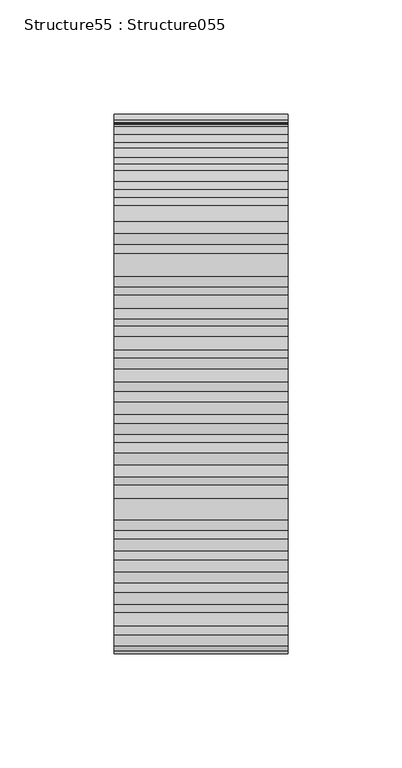
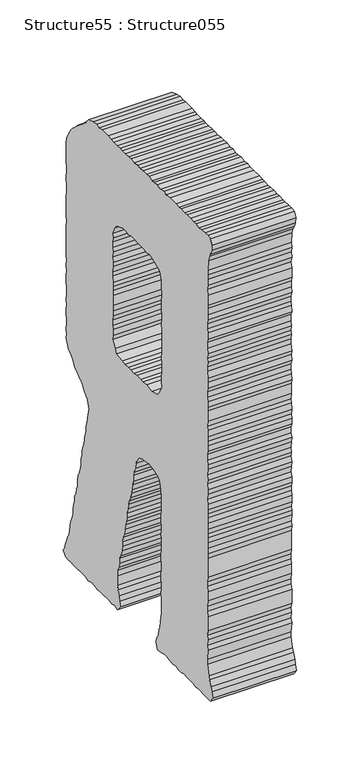
"""IFC4 building model written with IfcOpenShell, lengths in millimetres: proxy geometry, Structure55 : Structure055."""

from ifc_helpers import new_model, si_unit, frame, origin, place, context, project, spatial, polyline, outline, extrude, source, transform, mapped, element, save


def structure55_structure055_96c68484(model_context):
    return source(origin(), model_context, "Body", "SweptSolid", [
        extrude(outline(polyline([(253600.0102866, 3899.7046941), (253600.0102866, 3894.4030808), (253600.6007811, 3890.320967), (253600.0102866, 3884.4609514), (253600.0102866, 3880.3627915), (253599.4262106, 3876.263027), (253600.6007811, 3870.4030114), (253600.0102866, 3866.8776953), (253600.0102866, 3856.9179152), (253600.6007811, 3851.6612309), (253600.0102866, 3846.9757858), (253600.0102866, 3842.8583706), (253599.4262106, 3838.1761347), (253600.6007811, 3832.8921721), (253599.4262106, 3827.6162325), (253600.0102866, 3823.5341187), (253600.6007811, 3818.2309008), (253599.4262106, 3810.0474179), (253599.4262106, 3804.1890069), (253600.6007811, 3800.0876378), (253599.4262106, 3794.8309535), (253600.6007811, 3790.7039107), (253600.6007811, 3785.4456218), (253599.4262106, 3781.9299333), (253599.4262106, 3777.2444882), (253600.6007811, 3771.3860772), (253599.4262106, 3766.684586), (253600.6007811, 3762.5848215), (253596.5026212, 3753.8012165), (253592.3932291, 3751.4424479), (253589.4680351, 3747.9428055), (253586.5428411, 3743.2332913), (253582.4430766, 3739.7416719), (253579.5098596, 3737.9750024), (253575.4084905, 3734.47536), (253571.892802, 3729.7738688), (253568.9579804, 3726.2742264), (253566.0327864, 3723.9154578), (253563.6916685, 3716.2887726), (253566.0327864, 3706.9130685), (253567.1993339, 3701.0723082), (253568.367486, 3696.9709391), (253568.367486, 3691.6869765), (253570.1341555, 3687.587212), (253571.308726, 3683.4858429), (253571.892802, 3678.2018803), (253573.6514486, 3674.1277895), (253574.8163914, 3670.0007467), (253575.4084905, 3665.3265338), (253576.5750379, 3660.6250426), (253576.5750379, 3654.7842823), (253578.9257835, 3646.557475), (253581.2685061, 3641.8832621), (253582.4430766, 3636.6153456), (253581.8493729, 3631.3410106), (253583.601601, 3627.8397636), (253584.1920955, 3622.555801), (253586.5428411, 3619.0385079), (253587.1188941, 3613.772196), (253588.2934646, 3609.6547808), (253589.4680351, 3604.3964919), (253589.4680351, 3600.2967274), (253590.6442102, 3595.5872132), (253592.9837235, 3590.3289243), (253594.1615032, 3585.0706354), (253595.9105221, 3576.2693797), (253598.2532447, 3572.7440636), (253599.4262106, 3568.0682461), (253601.1848571, 3564.54293), (253602.3530092, 3559.2669905), (253604.7021502, 3556.3417965), (253601.1848571, 3551.6675836), (253596.5026212, 3551.0658569), (253592.9837235, 3551.6675836), (253588.2934646, 3551.0658569), (253583.0271526, 3551.0658569), (253578.3336845, 3551.6675836), (253569.5404518, 3551.6675836), (253565.4406874, 3550.4833855), (253559.5822763, 3551.6675836), (253556.0730063, 3551.6675836), (253551.3795382, 3550.4833855), (253545.5307548, 3551.0658569), (253532.0472632, 3551.0658569), (253527.9458941, 3550.4833855), (253523.836502, 3551.6675836), (253519.1606845, 3550.4833855), (253514.4704255, 3556.3417965), (253516.2194444, 3560.441561), (253516.8115435, 3565.1254015), (253517.986114, 3570.4109687), (253519.1606845, 3573.9266571), (253519.1606845, 3583.2863152), (253519.1606845, 3588.5702778), (253516.8115435, 3592.6700423), (253516.2194444, 3596.7698067), (253515.644996, 3602.0280957), (253513.2958551, 3606.1551384), (253512.1180754, 3611.4134274), (253511.5436269, 3616.0972679), (253510.9531325, 3620.7971545), (253510.3690565, 3625.472972), (253508.0263339, 3629.5984101), (253507.4454671, 3634.856699), (253506.8517634, 3639.5405396), (253505.0947215, 3644.2420307), (253503.928174, 3648.3161216), (253503.928174, 3652.4431643), (253502.7519989, 3657.7014533), (253501.5774284, 3662.3836892), (253499.8284095, 3667.0851803), (253498.6426068, 3670.5848228), (253496.8919833, 3675.8687854), (253496.3111165, 3679.9701544), (253495.1349414, 3685.2444894), (253493.9603709, 3689.3458585), (253493.9603709, 3695.2122926), (253492.7922188, 3698.711935), (253491.0255493, 3703.4134261), (253489.8509788, 3709.2718371), (253485.7496097, 3716.8985223), (253478.7246512, 3719.8140887), (253472.8662402, 3719.8140887), (253469.3585748, 3720.9726131), (253463.4905361, 3719.8140887), (253455.2894025, 3717.4729707), (253452.3561855, 3713.9556777), (253450.6071666, 3706.9130685), (253449.4293869, 3701.6547796), (253449.4293869, 3688.1873341), (253450.6071666, 3683.4858429), (253450.6071666, 3677.6274319), (253449.4293869, 3672.9435914), (253450.013463, 3668.2437048), (253450.6071666, 3664.7440624), (253450.013463, 3660.0682449), (253450.013463, 3654.1841602), (253449.4293869, 3650.1004418), (253450.6071666, 3644.8245022), (253450.6071666, 3640.114988), (253450.013463, 3636.6153456), (253449.4293869, 3631.915459), (253450.6071666, 3626.0554434), (253450.6071666, 3621.3732075), (253449.4293869, 3617.2718384), (253449.4293869, 3613.1720739), (253450.6071666, 3607.8961343), (253449.4293869, 3602.6298224), (253450.013463, 3597.9540049), (253450.013463, 3594.4286888), (253449.4293869, 3589.1527492), (253450.6071666, 3585.0706354), (253451.7817371, 3574.5107332), (253453.530756, 3570.9854171), (253454.7069311, 3565.1254015), (253457.0480491, 3561.6257591), (253458.2242242, 3556.3417965), (253455.8734786, 3550.4833855), (253450.013463, 3551.0658569), (253445.331227, 3552.242032), (253441.2218349, 3552.242032), (253437.1204658, 3551.6675836), (253431.8557585, 3551.0658569), (253427.1622903, 3551.6675836), (253423.0609212, 3551.0658569), (253418.3690577, 3551.0658569), (253414.2773162, 3552.242032), (253409.5838481, 3551.6675836), (253399.6272772, 3551.6675836), (253394.9418321, 3551.0658569), (253390.8420676, 3551.6675836), (253380.8758691, 3551.6675836), (253376.7841276, 3551.0658569), (253372.6827585, 3551.0658569), (253368.5733664, 3556.3417965), (253370.3223853, 3561.6257591), (253371.508188, 3565.7094775), (253373.8396783, 3570.9854171), (253375.0158534, 3574.5107332), (253377.358576, 3583.8864372), (253377.358576, 3588.5702778), (253376.1904239, 3597.9540049), (253377.358576, 3602.0280957), (253376.7841276, 3607.8961343), (253377.358576, 3612.0135494), (253376.1904239, 3616.69739), (253376.1904239, 3630.1824862), (253377.358576, 3634.856699), (253377.358576, 3639.5405396), (253376.7841276, 3645.4262289), (253376.7841276, 3654.1841602), (253377.358576, 3658.8840468), (253377.358576, 3663.5598643), (253376.7841276, 3668.2437048), (253376.7841276, 3686.4030139), (253376.1904239, 3691.0868544), (253376.7841276, 3695.786741), (253376.1904239, 3701.6547796), (253376.1904239, 3706.3289925), (253376.7841276, 3709.8559132), (253376.1904239, 3714.5301261), (253376.1904239, 3720.4158154), (253376.7841276, 3725.0996559), (253376.7841276, 3729.1737467), (253376.1904239, 3733.2991849), (253376.1904239, 3738.5574738), (253377.358576, 3742.6748889), (253376.7841276, 3747.9428055), (253376.1904239, 3752.6170184), (253377.358576, 3757.8753073), (253376.7841276, 3761.418274), (253377.358576, 3766.1021146), (253376.7841276, 3771.9605256), (253376.1904239, 3776.6427615), (253377.358576, 3780.1616592), (253377.358576, 3786.0280932), (253376.1904239, 3789.5293402), (253376.1904239, 3794.8309535), (253376.7841276, 3798.9050443), (253376.1904239, 3803.5872802), (253376.7841276, 3809.4729695), (253377.358576, 3812.9726119), (253376.7841276, 3818.2309008), (253376.7841276, 3828.2163546), (253376.1904239, 3831.732043), (253376.7841276, 3836.9919366), (253377.358576, 3841.0900965), (253377.358576, 3846.3772683), (253376.1904239, 3850.4754282), (253376.7841276, 3855.7353217), (253376.1904239, 3859.8591552), (253377.358576, 3865.7015202), (253377.358576, 3870.4030114), (253376.7841276, 3875.0772243), (253377.358576, 3878.5784713), (253376.7841276, 3883.2863809), (253377.358576, 3887.9621984), (253377.358576, 3893.822214), (253376.1904239, 3897.3475301), (253376.7841276, 3903.2059411), (253377.358576, 3906.7328618), (253377.358576, 3911.4054701), (253376.1904239, 3916.0909152), (253376.7841276, 3920.7908018), (253376.7841276, 3926.6492128), (253376.1904239, 3930.1745289), (253376.1904239, 3939.5325823), (253377.358576, 3944.8165449), (253376.1904239, 3949.4923624), (253376.7841276, 3954.7506513), (253376.1904239, 3959.4617701), (253376.7841276, 3963.5615346), (253375.6063479, 3973.5197101), (253374.4317774, 3978.2035506), (253372.0906594, 3981.7208437), (253370.3223853, 3986.4046842), (253369.7415185, 3991.6806238), (253372.0906594, 3996.390138), (253376.7841276, 3996.9645864), (253380.8758691, 3996.9645864), (253386.7406985, 3996.390138), (253390.2515731, 3996.390138), (253395.5355357, 3996.9645864), (253399.6272772, 3996.390138), (253404.3095131, 3996.9645864), (253409.5838481, 3996.9645864), (253413.6932402, 3996.390138), (253418.9627614, 3996.9645864), (253422.4784498, 3996.390138), (253427.1622903, 3996.9645864), (253436.5460174, 3996.9645864), (253442.3964054, 3996.390138), (253445.9136985, 3997.5486624), (253451.1880334, 3996.390138), (253456.45595, 3997.5486624), (253461.1478136, 3996.9645864), (253464.6651066, 3996.390138), (253469.3585748, 3997.5486624), (253473.4583392, 3996.9645864), (253478.7246512, 3997.5486624), (253483.4068871, 3996.9645864), (253487.5162792, 3997.5486624), (253493.3666672, 3996.390138), (253498.0601354, 3996.9645864), (253501.5774284, 3996.9645864), (253507.4454671, 3996.390138), (253512.1180754, 3996.390138), (253515.0625246, 3996.9645864), (253519.7367375, 3996.390138), (253525.6047761, 3996.390138), (253529.1124416, 3996.9645864), (253533.8059097, 3997.5486624), (253543.7656898, 3997.5486624), (253547.8638497, 3996.9645864), (253552.5573179, 3997.5486624), (253557.8236298, 3996.390138), (253564.8469837, 3994.0233463), (253568.367486, 3989.9460463), (253571.892802, 3987.0048063), (253575.4084905, 3982.8793681), (253580.0827034, 3979.9621971), (253583.0271526, 3977.6194746), (253585.950742, 3974.1214368), (253590.0601341, 3970.5768654), (253592.3932291, 3967.6789497), (253595.9105221, 3962.9774586), (253599.4262106, 3955.360401), (253600.0102866, 3951.2606365), (253600.0102866, 3941.8753048), (253600.6007811, 3936.0345445), (253600.6007811, 3932.4899731), (253599.4262106, 3927.8077372), (253599.4262106, 3923.1319197), (253600.6007811, 3918.4480792), (253599.4262106, 3907.888177), (253599.4262106, 3903.2059411), (253600.0102866, 3899.7046941)]), holes=[polyline([(253472.8662402, 3794.8309535), (253478.7246512, 3794.2292268), (253482.2323166, 3794.8309535), (253488.1003553, 3794.8309535), (253493.3666672, 3793.6451507), (253498.0601354, 3794.2292268), (253501.5774284, 3794.2292268), (253507.4454671, 3793.6451507), (253511.5436269, 3794.8309535), (253520.3288366, 3795.960595), (253522.0874831, 3800.0876378), (253526.1872476, 3806.5317294), (253525.6047761, 3810.6298893), (253525.6047761, 3816.4883003), (253526.1872476, 3820.015221), (253526.1872476, 3825.2911606), (253525.6047761, 3829.374879), (253525.6047761, 3834.0474873), (253525.0110725, 3839.9331766), (253525.0110725, 3849.3008577), (253525.6047761, 3854.0007442), (253525.0110725, 3858.1021133), (253525.0110725, 3862.2018778), (253526.1872476, 3867.4601667), (253526.1872476, 3871.5599312), (253525.6047761, 3876.8438938), (253525.6047761, 3880.9452629), (253526.1872476, 3885.6210804), (253525.6047761, 3890.905043), (253526.1872476, 3895.0048075), (253526.1872476, 3900.2887701), (253525.6047761, 3904.3901392), (253526.1872476, 3908.46423), (253523.252426, 3915.5068392), (253519.7367375, 3919.0321552), (253510.9531325, 3922.5494483), (253506.2596643, 3922.5494483), (253502.7519989, 3921.3748778), (253498.0601354, 3922.5494483), (253483.4068871, 3922.5494483), (253477.5564991, 3921.9733953), (253474.0408107, 3921.3748778), (253469.3585748, 3922.5494483), (253464.6651066, 3921.3748778), (253456.45595, 3918.4480792), (253452.9482846, 3916.0909152), (253450.6071666, 3909.0627475), (253450.6071666, 3904.9645876), (253449.4293869, 3894.4030808), (253450.6071666, 3890.320967), (253450.6071666, 3880.3627915), (253449.4293869, 3876.8438938), (253450.013463, 3871.5599312), (253450.6071666, 3867.4601667), (253449.4293869, 3861.6178018), (253450.013463, 3858.1021133), (253450.013463, 3839.9331766), (253450.6071666, 3834.6588416), (253449.4293869, 3830.5574726), (253449.4293869, 3825.849563), (253450.013463, 3820.5896694), (253450.6071666, 3816.4883003), (253450.6071666, 3811.7884138), (253450.013463, 3805.9476534), (253452.9482846, 3800.0876378), (253455.8734786, 3795.960595), (253464.6651066, 3793.6451507), (253472.8662402, 3794.8309535)])]), frame((-38594.2176606, 0.0, 0.0), z_axis=(1.0, 0.0, 0.0), x_axis=(0.0, 1.0, 0.0)), (0.0, 0.0, 1.0), 76.2),
    ])


if __name__ == "__main__":
    model = new_model("IFC4")
    model_context = context("Model", 3, world=origin())
    ifc_project = project(units=[si_unit("LENGTHUNIT", "METRE", prefix="MILLI")], contexts=[model_context])
    site = spatial("IfcSite", under=ifc_project)
    building = spatial("IfcBuilding", under=site)
    placement = place(None, origin())
    structure55_structure055_shape = structure55_structure055_96c68484(model_context)
    element("IfcBuildingElementProxy", 1, Name="Structure55 : Structure055", ObjectType="Structure55 : Structure055", at=placement, inside=building, context=model_context, shape_type="MappedRepresentation", body=[
        mapped(structure55_structure055_shape, transform((0.0, 0.0, 0.0), x_axis=(1.0, 0.0, 0.0), y_axis=(0.0, 1.0, 0.0), z_axis=(0.0, 0.0, 1.0))),
    ])
    save(model, "model.ifc")

# Revit data of these elements
# Type "Structure55 : Structure055"
#   NameOverride = "Structure055"
# Element 1 (IfcBuildingElementProxy, "Structure55 : Structure055")
#   Materials on its faces: "BRUSHED ALUM. LETTERING"
# Materials
#   "BRUSHED ALUM. LETTERING": class "Unassigned", colour RGB 169 181 186, transparency 0, Cost = 0
